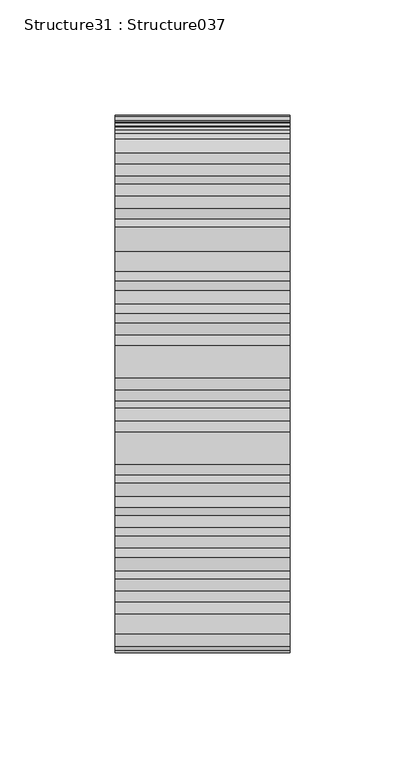
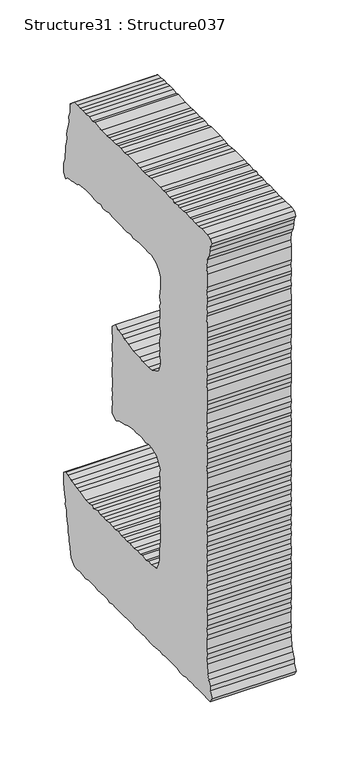
"""IFC4 building model written with IfcOpenShell, lengths in millimetres: proxy geometry, Structure31 : Structure037."""

import ifcopenshell
import ifcopenshell.guid

model = None  # the IFC model being written
_history = None  # IfcOwnerHistory: only IFC2X3 demands one
_inside = {}  # id of a spatial element -> (the spatial element, [elements in it])
_under = {}  # id of a project, library or spatial element -> (it, [spatial elements below it])
_declared = {}  # id of a project -> (the project, [libraries it declares])
_typed = {}  # id of a type object -> (the type object, [elements of that type])
_made_of = {}  # id of a material, layer set ... -> (it, [elements and type objects made of it])


def new_model(schema):
    """Start an empty IFC model of exactly this schema.

    Asked for "IFC4X3", IfcOpenShell would pick the latest addendum, in which some entities
    have other attributes; the version numbers below select the first issue.
    IFC2X3 requires an IfcOwnerHistory on every rooted entity: one is made here for all.
    """
    global model, _history
    if schema == "IFC4X3":
        model = ifcopenshell.file(schema_version=(4, 3, 0, 0))
    else:
        model = ifcopenshell.file(schema=schema)
    _inside.clear()
    _under.clear()
    _declared.clear()
    _typed.clear()
    _made_of.clear()
    _history = None
    if model.schema == "IFC2X3":
        org = make("IfcOrganization", Name="unknown")
        user = make(
            "IfcPersonAndOrganization",
            ThePerson=make("IfcPerson", FamilyName="unknown"),
            TheOrganization=org,
        )
        app = make(
            "IfcApplication",
            ApplicationDeveloper=org,
            Version="unknown",
            ApplicationFullName="unknown",
            ApplicationIdentifier="unknown",
        )
        _history = make(
            "IfcOwnerHistory",
            OwningUser=user,
            OwningApplication=app,
            ChangeAction="ADDED",
            CreationDate=0,
        )
    return model


def make(cls, **values):
    """One entity of the class cls with the attributes given. An attribute that is None is left unset."""
    return model.create_entity(
        cls, **{name: value for name, value in values.items() if value is not None}
    )


def rooted(cls, **values):
    """An entity with a GlobalId (a new one), such as an element, a storey or a relation."""
    return make(cls, GlobalId=ifcopenshell.guid.new(), OwnerHistory=_history, **values)


def si_unit(unit_type, name, prefix=None):
    """IfcSIUnit, for example si_unit("LENGTHUNIT", "METRE", prefix="MILLI")."""
    return make("IfcSIUnit", UnitType=unit_type, Prefix=prefix, Name=name)


def assignment(units):
    """IfcUnitAssignment: the units of a project."""
    return None if units is None else make("IfcUnitAssignment", Units=units)


def point(xyz):
    """IfcCartesianPoint."""
    return None if xyz is None else make("IfcCartesianPoint", Coordinates=xyz)


def direction(xyz):
    """IfcDirection."""
    return None if xyz is None else make("IfcDirection", DirectionRatios=xyz)


def frame(location, z_axis=None, x_axis=None):
    """IfcAxis2Placement3D, a coordinate frame: its origin and axes. An axis left out is left unset."""
    return make(
        "IfcAxis2Placement3D",
        Location=point(location),
        Axis=direction(z_axis),
        RefDirection=direction(x_axis),
    )


def origin():
    """The frame at (0, 0, 0) with its axes left unset."""
    return frame((0.0, 0.0, 0.0))


def place(relative_to, where):
    """IfcLocalPlacement: puts the frame where relative to a parent placement (None: the world)."""
    return make(
        "IfcLocalPlacement", PlacementRelTo=relative_to, RelativePlacement=where
    )


def context(
    kind, dimensions, precision=None, world=None, true_north=None, identifier=None
):
    """IfcGeometricRepresentationContext, for example the 3D "Model" context."""
    return make(
        "IfcGeometricRepresentationContext",
        ContextIdentifier=identifier,
        ContextType=kind,
        CoordinateSpaceDimension=dimensions,
        Precision=precision,
        WorldCoordinateSystem=world,
        TrueNorth=true_north,
    )


def project(units=None, contexts=None):
    """IfcProject with its units and contexts."""
    return rooted(
        "IfcProject",
        Name="project",
        RepresentationContexts=contexts,
        UnitsInContext=assignment(units),
    )


def spatial(cls, under=None, at=None, **own):
    """A site, building, storey or space (cls), placed at a placement, below another one or the project."""
    s = rooted(cls, ObjectPlacement=at, **own)
    if under is not None:
        _under.setdefault(under.id(), (under, []))[1].append(s)
    return s


def polyline(points):
    """IfcPolyline through the points."""
    return make("IfcPolyline", Points=[point(p) for p in points])


def outline(outer, holes=None, kind="AREA"):
    """IfcArbitraryClosedProfileDef: a profile drawn as a closed curve; with holes, ...WithVoids."""
    if holes is None:
        return make("IfcArbitraryClosedProfileDef", ProfileType=kind, OuterCurve=outer)
    return make(
        "IfcArbitraryProfileDefWithVoids",
        ProfileType=kind,
        OuterCurve=outer,
        InnerCurves=holes,
    )


def extrude(swept, where, along, depth):
    """IfcExtrudedAreaSolid: the profile swept, set in the frame where, extruded along a direction by depth."""
    return make(
        "IfcExtrudedAreaSolid",
        SweptArea=swept,
        Position=where,
        ExtrudedDirection=direction(along),
        Depth=depth,
    )


def shape(context_of_items, identifier, shape_type, items):
    """IfcShapeRepresentation: the items that make up one representation, for example the "Body"."""
    return make(
        "IfcShapeRepresentation",
        ContextOfItems=context_of_items,
        RepresentationIdentifier=identifier,
        RepresentationType=shape_type,
        Items=items,
    )


def source(mapping_origin, context_of_items, identifier, shape_type, items):
    """IfcRepresentationMap: a shape defined once, which mapped items show again and again."""
    return make(
        "IfcRepresentationMap",
        MappingOrigin=mapping_origin,
        MappedRepresentation=shape(context_of_items, identifier, shape_type, items),
    )


def transform(
    local_origin,
    x_axis=None,
    y_axis=None,
    z_axis=None,
    scale=None,
    scale2=None,
    scale3=None,
    uniform=True,
):
    """IfcCartesianTransformationOperator3D, or its non-uniform kind. x_axis, y_axis, z_axis: its Axis1, 2, 3."""
    if uniform:
        return make(
            "IfcCartesianTransformationOperator3D",
            Axis1=direction(x_axis),
            Axis2=direction(y_axis),
            LocalOrigin=point(local_origin),
            Scale=scale,
            Axis3=direction(z_axis),
        )
    return make(
        "IfcCartesianTransformationOperator3DnonUniform",
        Axis1=direction(x_axis),
        Axis2=direction(y_axis),
        LocalOrigin=point(local_origin),
        Scale=scale,
        Axis3=direction(z_axis),
        Scale2=scale2,
        Scale3=scale3,
    )


def mapped(mapping_source, mapping_target):
    """IfcMappedItem: shows the shape of a source again, moved by a transform."""
    return make(
        "IfcMappedItem", MappingSource=mapping_source, MappingTarget=mapping_target
    )


def made_of(thing, what):
    """Note that an element or type object is made of a material, layer set ...; save() writes the relation."""
    if what is not None:
        _made_of.setdefault(what.id(), (what, []))[1].append(thing)
    return thing


def element(
    cls,
    number,
    at=None,
    inside=None,
    cuts=None,
    type_object=None,
    material=None,
    context=None,
    identifier="Body",
    shape_type=None,
    held_by="IfcProductDefinitionShape",
    body=None,
    shapes=None,
    **own,
):
    """One element of the class cls, such as IfcWall. Its Tag is "e" and its number.

    at: its placement. inside: the storey or other place that contains it. cuts: it is an
    opening in that element (IfcRelVoidsElement). A single representation is given by context,
    identifier, shape_type and body (its items); several are given by shapes. held_by: the class
    of the entity that holds the representations. save() writes the other relations.
    """
    e = rooted(cls, Tag="e%d" % number, ObjectPlacement=at, **own)
    if body is not None:
        shapes = [shape(context, identifier, shape_type, body)]
    if shapes is not None:
        e.Representation = make(held_by, Representations=shapes)
    if inside is not None:
        _inside.setdefault(inside.id(), (inside, []))[1].append(e)
    if cuts is not None:
        rooted(
            "IfcRelVoidsElement", RelatingBuildingElement=cuts, RelatedOpeningElement=e
        )
    if type_object is not None:
        _typed.setdefault(type_object.id(), (type_object, []))[1].append(e)
    return made_of(e, material)


def aggregate(whole, parts):
    """IfcRelAggregates: a whole, such as a stair, and the parts it consists of."""
    return rooted("IfcRelAggregates", RelatingObject=whole, RelatedObjects=parts)


def save(model, path):
    """Write the relations noted so far, then the file.

    IfcRelAggregates (storeys below a building ...), IfcRelContainedInSpatialStructure (elements
    in a storey), IfcRelDefinesByType, IfcRelAssociatesMaterial and IfcRelDeclares: one each for
    every whole, place, type object, material and project.
    """
    for whole, parts in _under.values():
        aggregate(whole, parts)
    for where, things in _inside.values():
        rooted(
            "IfcRelContainedInSpatialStructure",
            RelatedElements=things,
            RelatingStructure=where,
        )
    for kind, things in _typed.values():
        rooted("IfcRelDefinesByType", RelatedObjects=things, RelatingType=kind)
    for what, things in _made_of.values():
        rooted("IfcRelAssociatesMaterial", RelatedObjects=things, RelatingMaterial=what)
    for by, libraries in _declared.values():
        rooted("IfcRelDeclares", RelatingContext=by, RelatedDefinitions=libraries)
    model.write(path)


def structure31_structure037_06b4eb6a(model_context):
    return source(origin(), model_context, "Body", "SweptSolid", [
        extrude(outline(polyline([(253294.767978, 3552.242032), (253291.2522896, 3551.0658569), (253285.97635, 3551.6675836), (253276.6006459, 3550.4833855), (253272.4992768, 3551.6675836), (253261.9570253, 3551.6675836), (253258.4397322, 3550.4833855), (253252.5716936, 3551.0658569), (253247.8894577, 3551.6675836), (253243.2040125, 3551.6675836), (253239.104248, 3550.4833855), (253234.4123845, 3551.6675836), (253229.7189164, 3551.0658569), (253215.6609764, 3551.0658569), (253212.1533109, 3551.6675836), (253202.7679792, 3551.6675836), (253197.5000627, 3550.4833855), (253193.4019028, 3551.0658569), (253188.7084347, 3551.0658569), (253183.4421227, 3551.6675836), (253179.9248296, 3551.0658569), (253174.6504947, 3550.4833855), (253170.5491256, 3550.4833855), (253159.9972464, 3551.6675836), (253155.8958773, 3551.0658569), (253151.2136414, 3551.6675836), (253133.0463093, 3551.6675836), (253128.3624688, 3550.4833855), (253123.6770237, 3550.4833855), (253118.9867647, 3551.6675836), (253114.8853956, 3551.0658569), (253110.1935321, 3551.6675836), (253104.3447487, 3551.0658569), (253100.2433796, 3551.6675836), (253090.8580479, 3551.6675836), (253085.5917359, 3551.0658569), (253080.8982678, 3551.0658569), (253077.9746784, 3555.7416744), (253080.8982678, 3561.6257591), (253081.4919715, 3565.7094775), (253083.2409904, 3570.9854171), (253085.0092645, 3575.6853037), (253086.1742074, 3583.8864372), (253086.7582834, 3588.5702778), (253086.1742074, 3593.8285667), (253086.7582834, 3597.9540049), (253086.7582834, 3607.3393366), (253086.1742074, 3612.0135494), (253086.7582834, 3616.69739), (253085.5917359, 3621.3732075), (253085.5917359, 3626.6571701), (253086.1742074, 3630.7392839), (253086.7582834, 3636.0408972), (253086.1742074, 3641.2991861), (253085.5917359, 3645.4262289), (253086.1742074, 3650.1004418), (253085.5917359, 3654.7842823), (253086.7582834, 3658.8840468), (253086.1742074, 3663.5598643), (253086.1742074, 3668.8261762), (253086.7582834, 3672.9435914), (253086.7582834, 3677.6274319), (253086.1742074, 3682.8857208), (253086.7582834, 3687.587212), (253086.1742074, 3692.2710525), (253086.7582834, 3696.3884676), (253085.5917359, 3701.6547796), (253086.1742074, 3706.9130685), (253086.7582834, 3710.4560353), (253085.5917359, 3715.1302482), (253086.7582834, 3720.4158154), (253086.1742074, 3725.0996559), (253085.5917359, 3730.3563402), (253086.7582834, 3733.8736333), (253086.1742074, 3739.1592005), (253085.5917359, 3743.2332913), (253086.7582834, 3748.5429276), (253086.1742074, 3753.2171405), (253086.1742074, 3762.5848215), (253085.5917359, 3767.8607611), (253086.7582834, 3771.3860772), (253085.5917359, 3777.2444882), (253085.5917359, 3781.3282066), (253086.1742074, 3786.6298199), (253085.5917359, 3791.3056374), (253086.7582834, 3795.960595), (253085.5917359, 3799.5051664), (253086.7582834, 3804.7730829), (253085.5917359, 3810.0474179), (253086.7582834, 3814.7296538), (253086.7582834, 3824.1149855), (253086.1742074, 3828.2163546), (253086.1742074, 3832.8921721), (253085.5917359, 3836.9919366), (253085.5917359, 3846.9757858), (253086.7582834, 3852.2340747), (253086.7582834, 3855.7353217), (253086.1742074, 3861.0192843), (253086.7582834, 3866.3032469), (253085.5917359, 3874.5043805), (253086.1742074, 3879.7610648), (253085.5917359, 3884.4609514), (253086.1742074, 3889.7208449), (253086.1742074, 3894.4030808), (253085.5917359, 3897.9476522), (253086.1742074, 3902.6314927), (253085.5917359, 3907.3313793), (253086.7582834, 3917.8479571), (253085.5917359, 3921.3748778), (253086.7582834, 3926.0490907), (253086.1742074, 3931.9058971), (253085.5917359, 3935.4328178), (253086.7582834, 3940.718385), (253085.5917359, 3945.9766739), (253085.5917359, 3958.8776941), (253086.7582834, 3964.1343784), (253085.5917359, 3972.3627903), (253082.6665419, 3977.6194746), (253082.0728383, 3982.8793681), (253080.8982678, 3987.5792547), (253079.1412259, 3991.6806238), (253080.8982678, 3995.7803883), (253086.1742074, 3996.390138), (253094.959417, 3996.390138), (253100.2433796, 3995.7803883), (253104.9256155, 3995.7803883), (253110.1935321, 3996.390138), (253113.7108251, 3995.7803883), (253119.5788638, 3996.9645864), (253123.6770237, 3995.7803883), (253128.9465448, 3996.390138), (253132.4622333, 3996.390138), (253137.7381728, 3995.7803883), (253141.2538613, 3996.9645864), (253145.9473294, 3995.7803883), (253151.7977174, 3996.9645864), (253155.3150105, 3996.390138), (253159.9972464, 3996.9645864), (253174.0664186, 3996.9645864), (253178.7486545, 3996.390138), (253184.6070656, 3995.7803883), (253187.5434918, 3995.7803883), (253192.2257277, 3996.390138), (253197.5000627, 3996.9645864), (253211.5612119, 3996.9645864), (253216.2514708, 3995.7803883), (253221.520992, 3996.9645864), (253225.6207565, 3996.9645864), (253229.7189164, 3995.7803883), (253235.586955, 3995.7803883), (253239.6883241, 3996.390138), (253243.7977162, 3995.7803883), (253252.5716936, 3995.7803883), (253263.1235727, 3996.9645864), (253266.6312382, 3995.7803883), (253271.3231017, 3996.9645864), (253276.6006459, 3996.9645864), (253281.8669579, 3996.390138), (253285.3842509, 3996.9645864), (253290.6585859, 3996.390138), (253295.352054, 3996.390138), (253301.2104651, 3991.6806238), (253301.2104651, 3988.1633307), (253301.2104651, 3983.4794902), (253303.551583, 3977.6194746), (253302.9691116, 3973.5197101), (253303.551583, 3969.994394), (253305.3102295, 3965.3201811), (253306.4864046, 3959.4617701), (253305.8943056, 3955.360401), (253307.0672715, 3951.2606365), (253308.2354235, 3946.5511223), (253308.2354235, 3942.4770315), (253308.8291272, 3937.1930689), (253309.409994, 3933.6741713), (253311.1686406, 3928.4158823), (253311.7527166, 3924.2888396), (253311.7527166, 3919.6066036), (253308.2354235, 3915.5068392), (253305.3102295, 3917.8479571), (253300.0439176, 3918.4480792), (253295.352054, 3919.6066036), (253290.6585859, 3920.2067257), (253287.7349965, 3922.5494483), (253277.1911404, 3923.7079727), (253267.8058087, 3923.7079727), (253263.7060442, 3922.5494483), (253258.4397322, 3922.5494483), (253253.7478687, 3923.7079727), (253249.0544005, 3922.5494483), (253244.954636, 3922.5494483), (253240.2724001, 3923.7079727), (253234.4123845, 3923.1319197), (253220.3528399, 3923.1319197), (253215.6609764, 3922.5494483), (253211.5612119, 3922.5494483), (253206.2948999, 3923.7079727), (253202.1935308, 3922.5494483), (253196.3254922, 3923.1319197), (253192.8098037, 3923.7079727), (253183.4421227, 3923.7079727), (253178.7486545, 3923.1319197), (253173.4743196, 3923.7079727), (253165.8556574, 3920.7908018), (253162.339969, 3916.6653636), (253159.414775, 3910.8310217), (253159.414775, 3900.2887701), (253159.9972464, 3896.763454), (253160.5893455, 3891.5067697), (253159.414775, 3886.2051565), (253160.5893455, 3883.2863809), (253159.9972464, 3878.5784713), (253159.9972464, 3873.3185778), (253160.5893455, 3868.0618934), (253160.5893455, 3863.9332461), (253159.414775, 3859.2606378), (253159.414775, 3855.1769193), (253160.5893455, 3849.8753061), (253160.5893455, 3845.8012153), (253159.9972464, 3840.5172527), (253160.5893455, 3835.8334121), (253159.414775, 3831.1575946), (253159.414775, 3827.6162325), (253162.339969, 3818.8310229), (253172.8822205, 3813.5743386), (253178.7486545, 3812.9726119), (253186.9594158, 3812.9726119), (253192.8098037, 3814.148787), (253202.1935308, 3814.148787), (253210.3866414, 3815.9154565), (253216.2514708, 3817.6741031), (253220.3528399, 3818.8310229), (253225.6207565, 3820.015221), (253230.31262, 3822.348316), (253235.0060882, 3818.2309008), (253235.586955, 3814.7296538), (253234.4123845, 3805.3459267), (253235.0060882, 3799.5051664), (253235.586955, 3795.960595), (253234.4123845, 3791.3056374), (253235.0060882, 3785.4456218), (253234.4123845, 3781.9299333), (253235.586955, 3776.6427615), (253235.586955, 3771.3860772), (253234.4123845, 3766.684586), (253234.4123845, 3762.0023501), (253235.0060882, 3757.8753073), (253234.4123845, 3753.8012165), (253235.586955, 3748.5429276), (253234.4123845, 3744.4158848), (253235.0060882, 3739.7416719), (253235.0060882, 3734.47536), (253229.1380495, 3730.9323932), (253225.0463081, 3733.2991849), (253220.944939, 3734.47536), (253215.0769003, 3735.6146291), (253210.3866414, 3737.400554), (253201.6014318, 3739.1592005), (253197.5000627, 3738.5574738), (253191.6352333, 3739.1592005), (253188.1163356, 3739.7416719), (253182.2659476, 3738.5574738), (253178.1677877, 3739.1592005), (253172.8822205, 3739.1592005), (253165.2715814, 3736.2163558), (253163.5145395, 3733.8736333), (253159.414775, 3726.2742264), (253160.5893455, 3722.7312597), (253159.9972464, 3716.8985223), (253159.9972464, 3712.2146818), (253159.414775, 3708.087639), (253160.5893455, 3704.0135482), (253160.5893455, 3699.3136616), (253159.414775, 3694.029699), (253159.414775, 3689.3458585), (253159.9972464, 3685.8285655), (253159.9972464, 3677.0449604), (253159.414775, 3671.7690209), (253159.414775, 3657.7014533), (253159.9972464, 3654.1841602), (253160.5893455, 3648.9258713), (253160.5893455, 3638.9580681), (253162.932068, 3631.915459), (253165.2715814, 3628.4158166), (253174.0664186, 3626.0554434), (253178.7486545, 3626.6571701), (253182.2659476, 3625.472972), (253188.1163356, 3626.6571701), (253191.6352333, 3625.472972), (253196.3254922, 3626.0554434), (253201.6014318, 3625.472972), (253207.4598428, 3626.6571701), (253212.1533109, 3625.472972), (253216.8355469, 3626.0554434), (253220.944939, 3625.472972), (253226.2032279, 3626.6571701), (253230.31262, 3625.472972), (253234.4123845, 3626.0554434), (253239.6883241, 3626.6571701), (253245.5467351, 3625.472972), (253249.6481042, 3626.0554434), (253254.3383631, 3625.472972), (253258.4397322, 3626.6571701), (253264.2901202, 3625.472972), (253267.8058087, 3626.6571701), (253272.4992768, 3625.472972), (253277.1911404, 3625.472972), (253286.5588214, 3627.8397636), (253291.2522896, 3628.4158166), (253295.352054, 3629.5984101), (253299.4534231, 3631.3410106), (253305.3102295, 3632.5155811), (253308.2354235, 3633.6821286), (253311.7527166, 3631.3410106), (253311.7527166, 3625.472972), (253311.7527166, 3620.7971545), (253310.5877737, 3617.2718384), (253310.0036977, 3611.4134274), (253308.2354235, 3606.7295868), (253308.8291272, 3602.6298224), (253306.4864046, 3598.5284533), (253307.0672715, 3593.8285667), (253305.8943056, 3588.5702778), (253304.135659, 3584.4689087), (253304.135659, 3578.6104977), (253302.9691116, 3574.5107332), (253302.9691116, 3570.4109687), (253301.2104651, 3565.7094775), (253300.618366, 3559.8671125), (253300.0439176, 3556.3417965), (253294.767978, 3552.242032)])), frame((-38594.2176606, 0.0, 0.0), z_axis=(1.0, 0.0, 0.0), x_axis=(0.0, 1.0, 0.0)), (0.0, 0.0, 1.0), 76.2),
    ])


if __name__ == "__main__":
    model = new_model("IFC4")
    model_context = context("Model", 3, world=origin())
    ifc_project = project(units=[si_unit("LENGTHUNIT", "METRE", prefix="MILLI")], contexts=[model_context])
    site = spatial("IfcSite", under=ifc_project)
    building = spatial("IfcBuilding", under=site)
    placement = place(None, origin())
    structure31_structure037_shape = structure31_structure037_06b4eb6a(model_context)
    element("IfcBuildingElementProxy", 1, Name="Structure31 : Structure037", ObjectType="Structure31 : Structure037", at=placement, inside=building, context=model_context, shape_type="MappedRepresentation", body=[
        mapped(structure31_structure037_shape, transform((0.0, 0.0, 0.0), x_axis=(1.0, 0.0, 0.0), y_axis=(0.0, 1.0, 0.0), z_axis=(0.0, 0.0, 1.0))),
    ])
    save(model, "model.ifc")

# Revit data of these elements
# Type "Structure31 : Structure037"
#   NameOverride = "Structure037"
# Element 1 (IfcBuildingElementProxy, "Structure31 : Structure037")
#   Materials on its faces: "BRUSHED ALUM. LETTERING"
# Materials
#   "BRUSHED ALUM. LETTERING": class "Unassigned", colour RGB 169 181 186, transparency 0, Cost = 0
